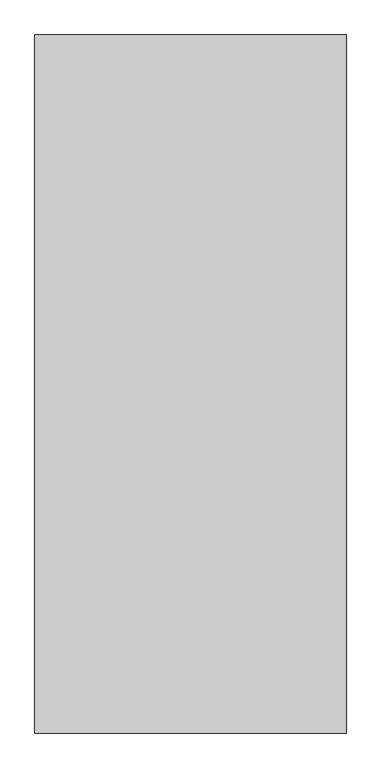
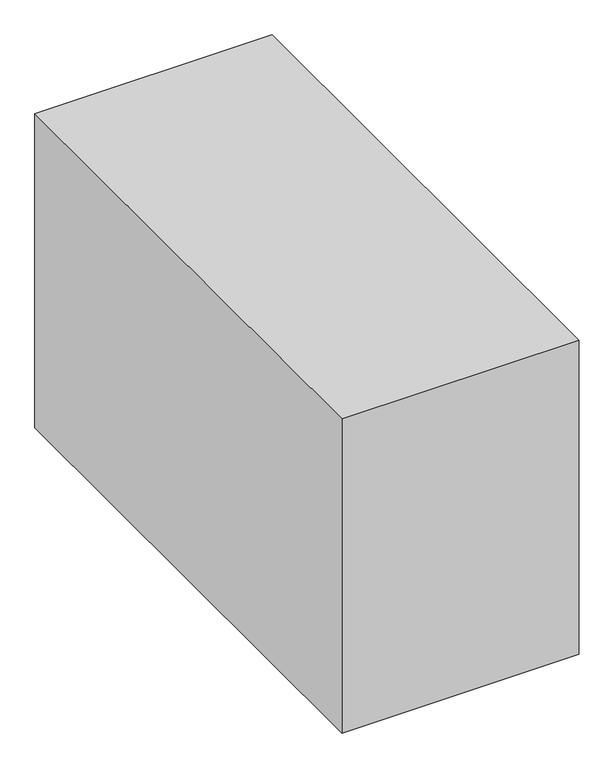
"""IFC4 building model written with IfcOpenShell, lengths in millimetres: proxy geometry, Space Planning Box_hec : Space Planning Box_hec."""

import ifcopenshell
import ifcopenshell.guid

model = None  # the IFC model being written
_history = None  # IfcOwnerHistory: only IFC2X3 demands one
_inside = {}  # id of a spatial element -> (the spatial element, [elements in it])
_under = {}  # id of a project, library or spatial element -> (it, [spatial elements below it])
_declared = {}  # id of a project -> (the project, [libraries it declares])
_typed = {}  # id of a type object -> (the type object, [elements of that type])
_made_of = {}  # id of a material, layer set ... -> (it, [elements and type objects made of it])


def new_model(schema):
    """Start an empty IFC model of exactly this schema.

    Asked for "IFC4X3", IfcOpenShell would pick the latest addendum, in which some entities
    have other attributes; the version numbers below select the first issue.
    IFC2X3 requires an IfcOwnerHistory on every rooted entity: one is made here for all.
    """
    global model, _history
    if schema == "IFC4X3":
        model = ifcopenshell.file(schema_version=(4, 3, 0, 0))
    else:
        model = ifcopenshell.file(schema=schema)
    _inside.clear()
    _under.clear()
    _declared.clear()
    _typed.clear()
    _made_of.clear()
    _history = None
    if model.schema == "IFC2X3":
        org = make("IfcOrganization", Name="unknown")
        user = make(
            "IfcPersonAndOrganization",
            ThePerson=make("IfcPerson", FamilyName="unknown"),
            TheOrganization=org,
        )
        app = make(
            "IfcApplication",
            ApplicationDeveloper=org,
            Version="unknown",
            ApplicationFullName="unknown",
            ApplicationIdentifier="unknown",
        )
        _history = make(
            "IfcOwnerHistory",
            OwningUser=user,
            OwningApplication=app,
            ChangeAction="ADDED",
            CreationDate=0,
        )
    return model


def make(cls, **values):
    """One entity of the class cls with the attributes given. An attribute that is None is left unset."""
    return model.create_entity(
        cls, **{name: value for name, value in values.items() if value is not None}
    )


def rooted(cls, **values):
    """An entity with a GlobalId (a new one), such as an element, a storey or a relation."""
    return make(cls, GlobalId=ifcopenshell.guid.new(), OwnerHistory=_history, **values)


def si_unit(unit_type, name, prefix=None):
    """IfcSIUnit, for example si_unit("LENGTHUNIT", "METRE", prefix="MILLI")."""
    return make("IfcSIUnit", UnitType=unit_type, Prefix=prefix, Name=name)


def assignment(units):
    """IfcUnitAssignment: the units of a project."""
    return None if units is None else make("IfcUnitAssignment", Units=units)


def point(xyz):
    """IfcCartesianPoint."""
    return None if xyz is None else make("IfcCartesianPoint", Coordinates=xyz)


def direction(xyz):
    """IfcDirection."""
    return None if xyz is None else make("IfcDirection", DirectionRatios=xyz)


def frame(location, z_axis=None, x_axis=None):
    """IfcAxis2Placement3D, a coordinate frame: its origin and axes. An axis left out is left unset."""
    return make(
        "IfcAxis2Placement3D",
        Location=point(location),
        Axis=direction(z_axis),
        RefDirection=direction(x_axis),
    )


def origin():
    """The frame at (0, 0, 0) with its axes left unset."""
    return frame((0.0, 0.0, 0.0))


def origin_with_axes():
    """The frame at (0, 0, 0) with the z axis (0, 0, 1) and the x axis (1, 0, 0) written out."""
    return frame((0.0, 0.0, 0.0), z_axis=(0.0, 0.0, 1.0), x_axis=(1.0, 0.0, 0.0))


def place(relative_to, where):
    """IfcLocalPlacement: puts the frame where relative to a parent placement (None: the world)."""
    return make(
        "IfcLocalPlacement", PlacementRelTo=relative_to, RelativePlacement=where
    )


def context(
    kind, dimensions, precision=None, world=None, true_north=None, identifier=None
):
    """IfcGeometricRepresentationContext, for example the 3D "Model" context."""
    return make(
        "IfcGeometricRepresentationContext",
        ContextIdentifier=identifier,
        ContextType=kind,
        CoordinateSpaceDimension=dimensions,
        Precision=precision,
        WorldCoordinateSystem=world,
        TrueNorth=true_north,
    )


def project(units=None, contexts=None):
    """IfcProject with its units and contexts."""
    return rooted(
        "IfcProject",
        Name="project",
        RepresentationContexts=contexts,
        UnitsInContext=assignment(units),
    )


def spatial(cls, under=None, at=None, **own):
    """A site, building, storey or space (cls), placed at a placement, below another one or the project."""
    s = rooted(cls, ObjectPlacement=at, **own)
    if under is not None:
        _under.setdefault(under.id(), (under, []))[1].append(s)
    return s


def polyline(points):
    """IfcPolyline through the points."""
    return make("IfcPolyline", Points=[point(p) for p in points])


def outline(outer, holes=None, kind="AREA"):
    """IfcArbitraryClosedProfileDef: a profile drawn as a closed curve; with holes, ...WithVoids."""
    if holes is None:
        return make("IfcArbitraryClosedProfileDef", ProfileType=kind, OuterCurve=outer)
    return make(
        "IfcArbitraryProfileDefWithVoids",
        ProfileType=kind,
        OuterCurve=outer,
        InnerCurves=holes,
    )


def extrude(swept, where, along, depth):
    """IfcExtrudedAreaSolid: the profile swept, set in the frame where, extruded along a direction by depth."""
    return make(
        "IfcExtrudedAreaSolid",
        SweptArea=swept,
        Position=where,
        ExtrudedDirection=direction(along),
        Depth=depth,
    )


def shape(context_of_items, identifier, shape_type, items):
    """IfcShapeRepresentation: the items that make up one representation, for example the "Body"."""
    return make(
        "IfcShapeRepresentation",
        ContextOfItems=context_of_items,
        RepresentationIdentifier=identifier,
        RepresentationType=shape_type,
        Items=items,
    )


def source(mapping_origin, context_of_items, identifier, shape_type, items):
    """IfcRepresentationMap: a shape defined once, which mapped items show again and again."""
    return make(
        "IfcRepresentationMap",
        MappingOrigin=mapping_origin,
        MappedRepresentation=shape(context_of_items, identifier, shape_type, items),
    )


def transform(
    local_origin,
    x_axis=None,
    y_axis=None,
    z_axis=None,
    scale=None,
    scale2=None,
    scale3=None,
    uniform=True,
):
    """IfcCartesianTransformationOperator3D, or its non-uniform kind. x_axis, y_axis, z_axis: its Axis1, 2, 3."""
    if uniform:
        return make(
            "IfcCartesianTransformationOperator3D",
            Axis1=direction(x_axis),
            Axis2=direction(y_axis),
            LocalOrigin=point(local_origin),
            Scale=scale,
            Axis3=direction(z_axis),
        )
    return make(
        "IfcCartesianTransformationOperator3DnonUniform",
        Axis1=direction(x_axis),
        Axis2=direction(y_axis),
        LocalOrigin=point(local_origin),
        Scale=scale,
        Axis3=direction(z_axis),
        Scale2=scale2,
        Scale3=scale3,
    )


def mapped(mapping_source, mapping_target):
    """IfcMappedItem: shows the shape of a source again, moved by a transform."""
    return make(
        "IfcMappedItem", MappingSource=mapping_source, MappingTarget=mapping_target
    )


def made_of(thing, what):
    """Note that an element or type object is made of a material, layer set ...; save() writes the relation."""
    if what is not None:
        _made_of.setdefault(what.id(), (what, []))[1].append(thing)
    return thing


def element(
    cls,
    number,
    at=None,
    inside=None,
    cuts=None,
    type_object=None,
    material=None,
    context=None,
    identifier="Body",
    shape_type=None,
    held_by="IfcProductDefinitionShape",
    body=None,
    shapes=None,
    **own,
):
    """One element of the class cls, such as IfcWall. Its Tag is "e" and its number.

    at: its placement. inside: the storey or other place that contains it. cuts: it is an
    opening in that element (IfcRelVoidsElement). A single representation is given by context,
    identifier, shape_type and body (its items); several are given by shapes. held_by: the class
    of the entity that holds the representations. save() writes the other relations.
    """
    e = rooted(cls, Tag="e%d" % number, ObjectPlacement=at, **own)
    if body is not None:
        shapes = [shape(context, identifier, shape_type, body)]
    if shapes is not None:
        e.Representation = make(held_by, Representations=shapes)
    if inside is not None:
        _inside.setdefault(inside.id(), (inside, []))[1].append(e)
    if cuts is not None:
        rooted(
            "IfcRelVoidsElement", RelatingBuildingElement=cuts, RelatedOpeningElement=e
        )
    if type_object is not None:
        _typed.setdefault(type_object.id(), (type_object, []))[1].append(e)
    return made_of(e, material)


def aggregate(whole, parts):
    """IfcRelAggregates: a whole, such as a stair, and the parts it consists of."""
    return rooted("IfcRelAggregates", RelatingObject=whole, RelatedObjects=parts)


def save(model, path):
    """Write the relations noted so far, then the file.

    IfcRelAggregates (storeys below a building ...), IfcRelContainedInSpatialStructure (elements
    in a storey), IfcRelDefinesByType, IfcRelAssociatesMaterial and IfcRelDeclares: one each for
    every whole, place, type object, material and project.
    """
    for whole, parts in _under.values():
        aggregate(whole, parts)
    for where, things in _inside.values():
        rooted(
            "IfcRelContainedInSpatialStructure",
            RelatedElements=things,
            RelatingStructure=where,
        )
    for kind, things in _typed.values():
        rooted("IfcRelDefinesByType", RelatedObjects=things, RelatingType=kind)
    for what, things in _made_of.values():
        rooted("IfcRelAssociatesMaterial", RelatedObjects=things, RelatingMaterial=what)
    for by, libraries in _declared.values():
        rooted("IfcRelDeclares", RelatingContext=by, RelatedDefinitions=libraries)
    model.write(path)


def generic_models_6c75c912(model_context):
    return source(origin(), model_context, "Body", "SweptSolid", [
        extrude(outline(polyline([(1250.0, 2800.0), (1250.0, -2800.0), (-1250.0, -2800.0), (-1250.0, 2800.0), (1250.0, 2800.0)])), origin_with_axes(), (0.0, 0.0, 1.0), 3500.0),
    ])


if __name__ == "__main__":
    model = new_model("IFC4")
    model_context = context("Model", 3, world=origin())
    ifc_project = project(units=[si_unit("LENGTHUNIT", "METRE", prefix="MILLI")], contexts=[model_context])
    site = spatial("IfcSite", under=ifc_project)
    building = spatial("IfcBuilding", under=site)
    placement = place(None, origin())
    generic_models_shape = generic_models_6c75c912(model_context)
    element("IfcBuildingElementProxy", 1, Name="Space Planning Box_hec : Space Planning Box_hec", ObjectType="Space Planning Box_hec : Space Planning Box_hec", at=placement, inside=building, context=model_context, shape_type="MappedRepresentation", body=[
        mapped(generic_models_shape, transform((0.0, 0.0, 0.0), x_axis=(1.0, 0.0, 0.0), y_axis=(0.0, 1.0, 0.0), z_axis=(0.0, 0.0, 1.0))),
    ])
    save(model, "model.ifc")

# Revit data of these elements
# Project information
#   Building Name = "MAIN GATE SECURITY BUILDING"
#   Project Status = "Project Status"
#   Client Name = "현대엔지니어링"
#   Project Address = "서울시 종로구 율곡로 75(계동)"
#   Project Name = "Therma Visayas Energy Project"
#   Project Number = "-"
# Type "Space Planning Box_hec : Space Planning Box_hec"
#   Type Comments = "..."
#   Room Name [instance default] = "?"
#   Interior Finish [instance default] = ""
#   Exterior Finish [instance default] = ""
#   Department [instance default] = ""
#   Assembly Code = "..."
#   Width [instance default] = 1524 mm
#   Program Area [instance default] = 0.00 m²
#   Length [instance default] = 1524 mm
#   Height [instance default] = 1524 mm
#   Area [instance default] = 2.32258 m²
#   Fill Color [instance default] = Cyan
#   Default Elevation = 0
# Element 1 (IfcBuildingElementProxy, "Space Planning Box_hec : Space Planning Box_hec")
#   Room Name = "Shower"
#   Width = 2500 mm
#   Program Area = 14.00 m²
#   Length = 5600 mm
#   Height = 3500 mm
#   Area = 14.00 m²
#   Materials on its faces: "Cyan"
# Materials
#   "Cyan": class "Generic", colour RGB 0 255 255, transparency 0.2, Cost = 0
